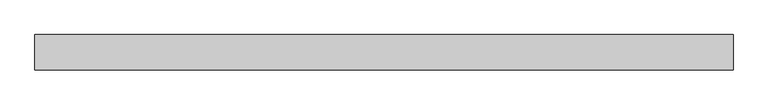
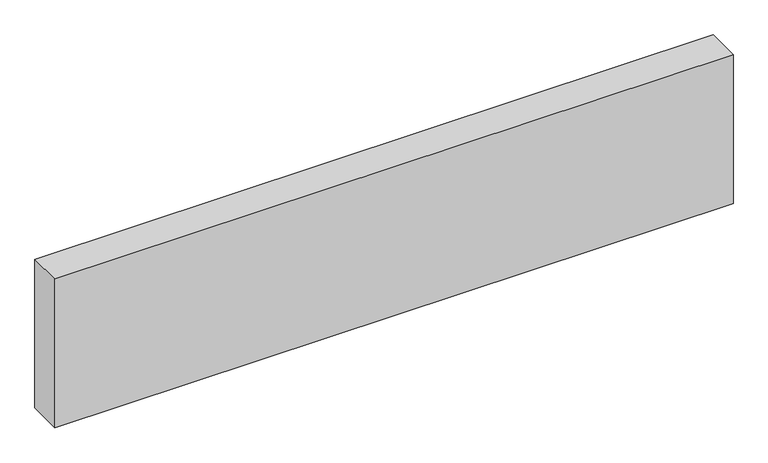
"""IFC4 building model written with IfcOpenShell, lengths in millimetres: proxy geometry, Generic Models 7:Generic Models 1:2:Generic Models 1:2 : Generic Models 7:Generic Models 1:337419:8 : Generic Models 7:Generic Models 1:2:Generic Models 1:2 : Generic Models 7:Generic Models 1:337419:306751."""

from ifc_helpers import new_model, si_unit, frame, origin, place, context, project, spatial, polyline, outline, extrude, source, transform, mapped, element, save


def generic_models_b6da56ad(model_context):
    return source(origin(), model_context, "Body", "SweptSolid", [
        extrude(outline(polyline([(596182.8367242, -536560.0694608), (596182.8367242, -536808.5132108), (591306.0367242, -536808.5132108), (591306.0367242, -536560.0694608), (596182.8367242, -536560.0694608)])), frame((0.0, 0.0, 2547.8106045), z_axis=(0.0, 0.0, 1.0), x_axis=(1.0, 0.0, 0.0)), (0.0, 0.0, 1.0), 1131.20164),
    ])


if __name__ == "__main__":
    model = new_model("IFC4")
    model_context = context("Model", 3, world=origin())
    ifc_project = project(units=[si_unit("LENGTHUNIT", "METRE", prefix="MILLI")], contexts=[model_context])
    site = spatial("IfcSite", under=ifc_project)
    building = spatial("IfcBuilding", under=site)
    placement = place(None, origin())
    generic_models_shape = generic_models_b6da56ad(model_context)
    element("IfcBuildingElementProxy", 1, Name="Generic Models 7:Generic Models 1:2:Generic Models 1:2 : Generic Models 7:Generic Models 1:337419:8 : Generic Models 7:Generic Models 1:2:Generic Models 1:2 : Generic Models 7:Generic Models 1:337419:306751", ObjectType="Generic Models 7:Generic Models 1:2:Generic Models 1:2 : Generic Models 7:Generic Models 1:337419:8 : Generic Models 7:Generic Models 1:2:Generic Models 1:2 : Generic Models 7:Generic Models 1:337419:306751", at=placement, inside=building, context=model_context, shape_type="MappedRepresentation", body=[
        mapped(generic_models_shape, transform((0.0, 0.0, 0.0), x_axis=(1.0, 0.0, 0.0), y_axis=(0.0, 1.0, 0.0), z_axis=(0.0, 0.0, 1.0))),
    ])
    save(model, "model.ifc")

# Revit data of these elements
# Type "Generic Models 7:Generic Models 1:2:Generic Models 1:2 : Generic Models 7:Generic Models 1:337419:8 : Generic Models 7:Generic Models 1:2:Generic Models 1:2 : Generic Models 7:Generic Models 1:337419:306751"
#   NameOverride = "Generic Models 7:Generic Models 1:2:Generic Models 1:2 : Generic Models 7:Generic Models 1:337419:306751"
#   ObjectTypeOverride = "Generic Models 1:2 : Generic Models 7:Generic Models 1:337419"
#   Reference = "Generic Models 1"
#   Tag = "306751"
# Element 1 (IfcBuildingElementProxy, "Generic Models 7:Generic Models 1:2:Generic Models 1:2 : Generic Models 7:Generic Models 1:337419:8 : Generic Models 7:Generic Models 1:2:Generic Models 1:2 : Generic Models 7:Generic Models 1:337419:306751")
#   Materials on its faces: "SIMPLE SAVER INSULATION WITH LINER - COLOR: BLACK"
# Materials
#   "SIMPLE SAVER INSULATION WITH LINER - COLOR: BLACK": class "Unassigned", colour RGB 158 92 175, transparency 0, Cost = 0
